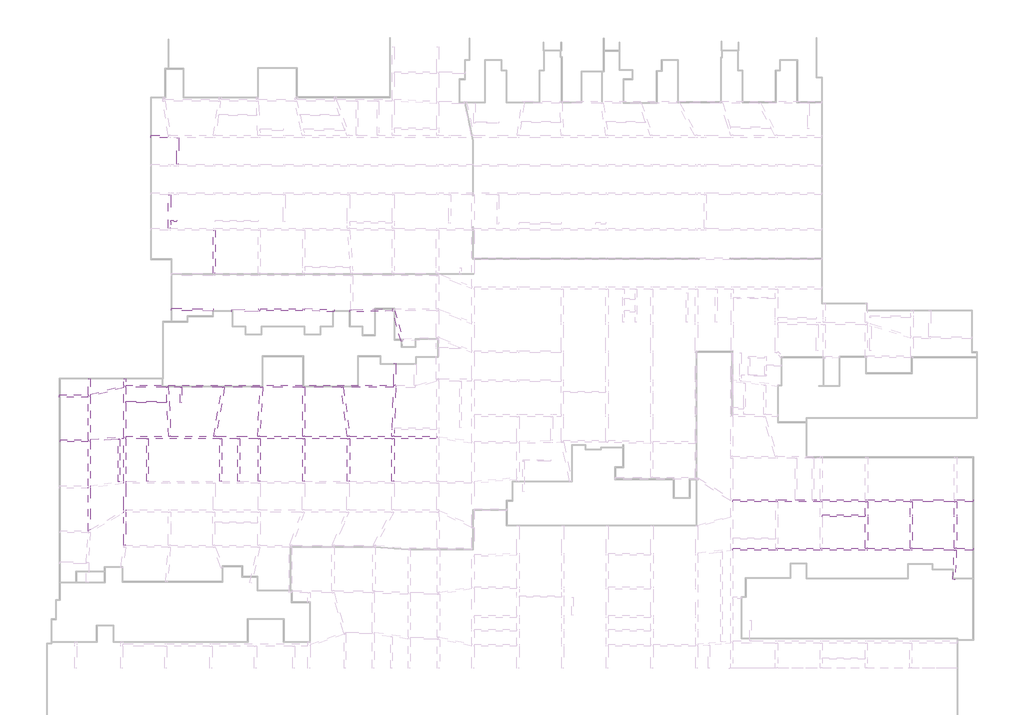
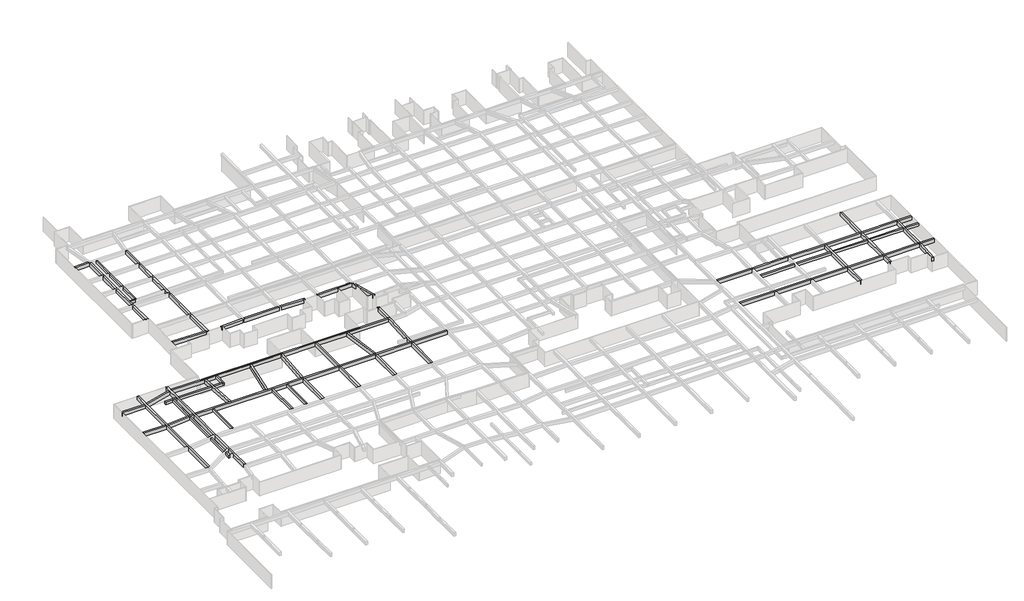
# One storey, part 11 of 16: 44 beams.
"""IFC4 building model written with IfcOpenShell, lengths in millimetres."""

from ifc_helpers import new_model, si_unit, frame, origin, place, context, project, spatial, polyline, outline, extrude, faceted_brep, element, save

model = new_model("IFC4")

# Units and contexts
model_context = context("Model", 3, world=origin())
ifc_project = project(units=[si_unit("LENGTHUNIT", "METRE", prefix="MILLI")], contexts=[model_context])

# Site, building, storey
site = spatial("IfcSite", under=ifc_project)
building = spatial("IfcBuilding", under=site)
storey = spatial("IfcBuildingStorey", under=building, Name="户型图", Elevation=0.0)

# Beams
placement = place(None, origin())
element("IfcBeam", 1, ObjectType="混凝土 - 矩形梁 : KL_beam", at=placement, inside=storey, context=model_context, shape_type="Brep", body=[
    faceted_brep([(83129.050114, 189895.7397162, 3300.0), (83129.050114, 190295.7397162, 3300.0), (83129.050114, 190295.7397162, 2500.0), (83129.050114, 189895.7397162, 2500.0), (86294.1615746, 189895.7397162, 3300.0), (86294.1615746, 190295.7397162, 3300.0), (86259.9916613, 190295.7397162, 3300.0), (86294.1615746, 190295.7397162, 2500.0), (86259.9916613, 190295.7397162, 2500.0), (86294.1615746, 189895.7397162, 2500.0)], [[[0, 1, 2, 3]], [[1, 0, 4, 5, 6]], [[2, 1, 6, 5, 7, 8]], [[3, 2, 8, 7, 9]], [[0, 3, 9, 4]], [[5, 4, 9, 7]]]),
])
element("IfcBeam", 2, ObjectType="混凝土 - 矩形梁 : KL_beam", at=placement, inside=storey, context=model_context, shape_type="Brep", body=[
    faceted_brep([(86694.1615746, 167850.6633594, 3300.0), (86294.1615746, 167850.6633594, 3300.0), (86294.1615746, 167850.6633594, 2500.0), (86694.1615746, 167850.6633594, 2500.0), (86694.1615746, 173112.5884701, 3300.0), (86294.1615746, 173112.5884701, 3300.0), (86294.1615746, 173112.5884701, 2500.0), (86694.1615746, 173112.5884701, 2500.0)], [[[0, 1, 2, 3]], [[1, 0, 4, 5]], [[2, 1, 5, 6]], [[3, 2, 6, 7]], [[0, 3, 7, 4]], [[5, 4, 7, 6]]]),
    faceted_brep([(86294.1615746, 189895.7397162, 3300.0), (86694.1615746, 189895.7397162, 3300.0), (86694.1615746, 189895.7397162, 2500.0), (86294.1615746, 189895.7397162, 2500.0), (86694.1615746, 185072.5884701, 3300.0), (86294.1615746, 185072.5884701, 3300.0), (86294.1615746, 185072.5884701, 2500.0), (86694.1615746, 185072.5884701, 2500.0)], [[[0, 1, 2, 3]], [[4, 5, 6, 7]], [[1, 0, 5, 4]], [[0, 3, 6, 5]], [[3, 2, 7, 6]], [[2, 1, 4, 7]]]),
    faceted_brep([(86294.1615746, 184672.5884701, 3300.0), (86694.1615746, 184672.5884701, 3300.0), (86694.1615746, 184672.5884701, 2500.0), (86294.1615746, 184672.5884701, 2500.0), (86694.1615746, 179912.5884701, 3300.0), (86294.1615746, 179912.5884701, 3300.0), (86294.1615746, 179912.5884701, 2500.0), (86694.1615746, 179912.5884701, 2500.0)], [[[0, 1, 2, 3]], [[4, 5, 6, 7]], [[1, 0, 5, 4]], [[0, 3, 6, 5]], [[3, 2, 7, 6]], [[2, 1, 4, 7]]]),
    faceted_brep([(86294.1615746, 179512.5884701, 3300.0), (86694.1615746, 179512.5884701, 3300.0), (86694.1615746, 179512.5884701, 2500.0), (86294.1615746, 179512.5884701, 2500.0), (86694.1615746, 173512.5884701, 3300.0), (86294.1615746, 173512.5884701, 3300.0), (86294.1615746, 173512.5884701, 2500.0), (86694.1615746, 173512.5884701, 2500.0), (86694.1615746, 174669.5403425, 3300.0), (86694.1615746, 174969.5403425, 3300.0)], [[[0, 1, 2, 3]], [[4, 5, 6, 7]], [[1, 0, 5, 4, 8, 9]], [[0, 3, 6, 5]], [[3, 2, 7, 6]], [[2, 1, 9, 8, 4, 7]]]),
])
element("IfcBeam", 3, ObjectType="混凝土 - 矩形梁 : KL_beam", at=placement, inside=storey, context=model_context, shape_type="Brep", body=[
    faceted_brep([(94416.2109037, 158476.0490175, 3300.0), (94816.2109037, 158476.0490175, 3300.0), (94816.2109037, 164912.5884701, 3300.0), (94416.2109037, 164912.5884701, 3300.0), (94416.2109037, 158876.1099487, 3300.0), (94416.2109037, 158476.0490175, 2500.0), (94416.2109037, 164912.5884701, 2500.0), (94416.2109037, 158876.1099487, 2500.0), (94816.2109037, 158476.0490175, 2500.0), (94816.2109037, 164912.5884701, 2500.0)], [[[0, 1, 2, 3, 4]], [[5, 0, 4, 3, 6, 7]], [[8, 5, 7, 6, 9]], [[1, 8, 9, 2]], [[3, 2, 9, 6]], [[1, 0, 5, 8]]]),
    faceted_brep([(94416.2109037, 189895.7397162, 3300.0), (94816.2109037, 189895.7397162, 3300.0), (94816.2109037, 189895.7397162, 2500.0), (94416.2109037, 189895.7397162, 2500.0), (94816.2109037, 185072.5884701, 3300.0), (94416.2109037, 185072.5884701, 3300.0), (94416.2109037, 185072.5884701, 2500.0), (94816.2109037, 185072.5884701, 2500.0)], [[[0, 1, 2, 3]], [[4, 5, 6, 7]], [[1, 0, 5, 4]], [[0, 3, 6, 5]], [[3, 2, 7, 6]], [[2, 1, 4, 7]]]),
    faceted_brep([(94416.2109037, 184672.5884701, 3300.0), (94816.2109037, 184672.5884701, 3300.0), (94816.2109037, 184672.5884701, 2500.0), (94416.2109037, 184672.5884701, 2500.0), (94816.2109037, 179912.5884701, 3300.0), (94416.2109037, 179912.5884701, 3300.0), (94416.2109037, 179912.5884701, 2500.0), (94816.2109037, 179912.5884701, 2500.0)], [[[0, 1, 2, 3]], [[4, 5, 6, 7]], [[1, 0, 5, 4]], [[0, 3, 6, 5]], [[3, 2, 7, 6]], [[2, 1, 4, 7]]]),
    faceted_brep([(94416.2109037, 179512.5884701, 3300.0), (94816.2109037, 179512.5884701, 3300.0), (94816.2109037, 179512.5884701, 2500.0), (94416.2109037, 179512.5884701, 2500.0), (94816.2109037, 173512.5884701, 3300.0), (94416.2109037, 173512.5884701, 3300.0), (94416.2109037, 173512.5884701, 2500.0), (94816.2109037, 173512.5884701, 2500.0), (94416.2109037, 174969.5403425, 3300.0), (94416.2109037, 174669.5403425, 3300.0), (94816.2109037, 174669.5403425, 3300.0), (94816.2109037, 174969.5403425, 3300.0)], [[[0, 1, 2, 3]], [[4, 5, 6, 7]], [[1, 0, 8, 9, 5, 4, 10, 11]], [[0, 3, 6, 5, 9, 8]], [[3, 2, 7, 6]], [[2, 1, 11, 10, 4, 7]]]),
    faceted_brep([(94416.2109037, 173112.5884701, 3300.0), (94816.2109037, 173112.5884701, 3300.0), (94816.2109037, 173112.5884701, 2500.0), (94416.2109037, 173112.5884701, 2500.0), (94816.2109037, 165312.5884701, 3300.0), (94416.2109037, 165312.5884701, 3300.0), (94416.2109037, 165312.5884701, 2500.0), (94816.2109037, 165312.5884701, 2500.0)], [[[0, 1, 2, 3]], [[4, 5, 6, 7]], [[1, 0, 5, 4]], [[0, 3, 6, 5]], [[3, 2, 7, 6]], [[2, 1, 4, 7]]]),
])
element("IfcBeam", 4, ObjectType="混凝土 - 矩形梁 : KL_beam", at=placement, inside=storey, context=model_context, shape_type="Brep", body=[
    faceted_brep([(86825.6773723, 158608.5422731, 3300.0), (86832.6583349, 159008.4813512, 3300.0), (86832.6583349, 159008.4813512, 2500.0), (86825.6773723, 158608.5422731, 2500.0), (94416.2109037, 158476.0490175, 3300.0), (94416.2109037, 158876.1099487, 3300.0), (94416.2109037, 158876.1099487, 2500.0), (94416.2109037, 158476.0490175, 2500.0), (94816.2109037, 158469.0669915, 2500.0), (94816.2109037, 158469.0669915, 3300.0), (94816.2109037, 158476.0490175, 2500.0), (94816.2109037, 158476.0490175, 3300.0)], [[[0, 1, 2, 3]], [[1, 0, 4, 5]], [[2, 1, 5, 6]], [[3, 2, 6, 7]], [[0, 3, 7, 8, 9, 4]], [[9, 8, 10, 11]], [[4, 7, 6, 5]], [[7, 4, 11, 10]], [[4, 9, 11]], [[10, 8, 7]]]),
])
element("IfcBeam", 5, ObjectType="混凝土 - 矩形梁 : KL_beam", at=placement, inside=storey, context=model_context, shape_type="SweptSolid", body=[
    extrude(outline(polyline([(97729.8525124, 158312.7245419), (97715.1918872, 158712.4557842), (102516.2109037, 158888.5389443), (102516.2109037, 158488.2700059), (97729.8525124, 158312.7245419)])), frame((0.0, 0.0, 2500.0), z_axis=(0.0, 0.0, 1.0), x_axis=(1.0, 0.0, 0.0)), (0.0, 0.0, 1.0), 800.0),
])
element("IfcBeam", 6, ObjectType="混凝土 - 矩形梁 : KL_beam", at=placement, inside=storey, context=model_context, shape_type="SweptSolid", body=[
    extrude(outline(polyline([(102916.2109037, 158502.9404881), (102916.2109037, 158895.7397162), (110616.2109037, 158895.7397162), (110616.2109037, 158495.7397162), (102719.8772917, 158495.7397162), (102916.2109037, 158502.9404881)])), frame((0.0, 0.0, 2500.0), z_axis=(0.0, 0.0, 1.0), x_axis=(1.0, 0.0, 0.0)), (0.0, 0.0, 1.0), 800.0),
])
element("IfcBeam", 7, ObjectType="混凝土 - 矩形梁 : KL_beam", at=placement, inside=storey, context=model_context, shape_type="SweptSolid", body=[
    extrude(outline(polyline([(116332.4791504, 158712.3385391), (116311.9369207, 158312.8663663), (111016.2109037, 158585.1907676), (111016.2109037, 158985.7192923), (116332.4791504, 158712.3385391)])), frame((0.0, 0.0, 2500.0), z_axis=(0.0, 0.0, 1.0), x_axis=(1.0, 0.0, 0.0)), (0.0, 0.0, 1.0), 800.0),
])
element("IfcBeam", 8, ObjectType="混凝土 - 矩形梁 : KL_beam", at=placement, inside=storey, context=model_context, shape_type="Brep", body=[
    faceted_brep([(119117.5153204, 158712.5269028, 3300.0), (119117.5153204, 158712.5269028, 2500.0), (119127.7719841, 158312.6584233, 2500.0), (119127.7719841, 158312.6584233, 3300.0), (126816.2109037, 158509.867597, 3300.0), (126816.2109037, 158909.9991608, 3300.0), (119689.6107616, 158727.2012041, 3300.0), (119289.6107616, 158716.9411668, 3300.0), (126816.2109037, 158509.867597, 2500.0), (119289.6107616, 158716.9411668, 2500.0), (119689.6107616, 158727.2012041, 2500.0), (126816.2109037, 158909.9991608, 2500.0)], [[[0, 1, 2, 3]], [[0, 3, 4, 5, 6, 7]], [[3, 2, 8, 4]], [[2, 1, 9, 10, 11, 8]], [[1, 0, 7, 6, 5, 11, 10, 9]], [[5, 4, 8, 11]]]),
])
element("IfcBeam", 9, ObjectType="混凝土 - 矩形梁 : KL_beam", at=placement, inside=storey, context=model_context, shape_type="Brep", body=[
    faceted_brep([(128438.9418632, 153027.8198438, 3300.0), (128848.9009007, 153049.3048866, 3300.0), (128735.7458004, 153443.9236175, 3300.0), (127281.619868, 158515.0633975, 3300.0), (127018.7754912, 158515.0633975, 3300.0), (126866.6192101, 158511.1605747, 3300.0), (126866.6192101, 158511.1605747, 2500.0), (128438.9418632, 153027.8198438, 2500.0), (128848.9009007, 153049.3048866, 2500.0), (127018.7754912, 158515.0633975, 2500.0), (127281.619868, 158515.0633975, 2500.0), (128735.7458004, 153443.9236175, 2500.0)], [[[0, 1, 2, 3, 4, 5]], [[5, 6, 7, 0]], [[8, 7, 6, 9, 10, 11]], [[1, 8, 11, 10, 3, 2]], [[6, 5, 4, 9]], [[4, 3, 10, 9]], [[1, 0, 7, 8]]]),
])
element("IfcBeam", 10, ObjectType="混凝土 - 矩形梁 : KL_beam", at=placement, inside=storey, context=model_context, shape_type="Brep", body=[
    faceted_brep([(232045.6960739, 124332.2101355, 3300.0), (232045.6960739, 123932.2101355, 3300.0), (232045.6960739, 123932.2101355, 2500.0), (232045.6960739, 124332.2101355, 2500.0), (229016.2421537, 124332.2101355, 3300.0), (228616.2421537, 124332.2101355, 3300.0), (221016.2265287, 124332.2101355, 3300.0), (220616.2265287, 124332.2101355, 3300.0), (212916.2109037, 124332.2101355, 3300.0), (212516.2109037, 124332.2101355, 3300.0), (204716.2109037, 124332.2101355, 3300.0), (204316.2109037, 124332.2101355, 3300.0), (203157.9308744, 124332.2101355, 3300.0), (202857.9308744, 124332.2101355, 3300.0), (200116.9298732, 124332.2101355, 3300.0), (199816.9298732, 124332.2101355, 3300.0), (196655.472134, 124332.2101355, 3300.0), (196255.472134, 124332.2101355, 3300.0), (188516.2109037, 124332.2101355, 3300.0), (188516.2109037, 123932.2101355, 3300.0), (196255.472134, 123932.2101355, 3300.0), (196655.472134, 123932.2101355, 3300.0), (204316.2109037, 123932.2101355, 3300.0), (204716.2109037, 123932.2101355, 3300.0), (212516.2109037, 123932.2101355, 3300.0), (212916.2109037, 123932.2101355, 3300.0), (220616.2265287, 123932.2101355, 3300.0), (221016.2265287, 123932.2101355, 3300.0), (228616.2421537, 123932.2101355, 3300.0), (229016.2421537, 123932.2101355, 3300.0), (188516.2109037, 123932.2101355, 2500.0), (196255.472134, 123932.2101355, 2500.0), (196655.472134, 123932.2101355, 2500.0), (204316.2109037, 123932.2101355, 2500.0), (204716.2109037, 123932.2101355, 2500.0), (212516.2109037, 123932.2101355, 2500.0), (212916.2109037, 123932.2101355, 2500.0), (220616.2265287, 123932.2101355, 2500.0), (221016.2265287, 123932.2101355, 2500.0), (228616.2421537, 123932.2101355, 2500.0), (229016.2421537, 123932.2101355, 2500.0), (188516.2109037, 124332.2101355, 2500.0), (196255.472134, 124332.2101355, 2500.0), (196655.472134, 124332.2101355, 2500.0), (204316.2109037, 124332.2101355, 2500.0), (204716.2109037, 124332.2101355, 2500.0), (212516.2109037, 124332.2101355, 2500.0), (212916.2109037, 124332.2101355, 2500.0), (220616.2265287, 124332.2101355, 2500.0), (221016.2265287, 124332.2101355, 2500.0), (228616.2421537, 124332.2101355, 2500.0), (229016.2421537, 124332.2101355, 2500.0)], [[[0, 1, 2, 3]], [[1, 0, 4, 5, 6, 7, 8, 9, 10, 11, 12, 13, 14, 15, 16, 17, 18, 19, 20, 21, 22, 23, 24, 25, 26, 27, 28, 29]], [[2, 1, 29, 28, 27, 26, 25, 24, 23, 22, 21, 20, 19, 30, 31, 32, 33, 34, 35, 36, 37, 38, 39, 40]], [[3, 2, 40, 39, 38, 37, 36, 35, 34, 33, 32, 31, 30, 41, 42, 43, 44, 45, 46, 47, 48, 49, 50, 51]], [[0, 3, 51, 50, 49, 48, 47, 46, 45, 44, 43, 42, 41, 18, 17, 16, 15, 14, 13, 12, 11, 10, 9, 8, 7, 6, 5, 4]], [[18, 41, 30, 19]]]),
])
element("IfcBeam", 11, ObjectType="混凝土 - 矩形梁 : KL_beam", at=placement, inside=storey, context=model_context, shape_type="Brep", body=[
    faceted_brep([(232047.570889, 115530.098028, 3300.0), (232047.570889, 115130.098028, 3300.0), (232047.570889, 115130.098028, 2500.0), (232047.570889, 115530.098028, 2500.0), (229016.2421537, 115530.098028, 3300.0), (228616.2421537, 115530.098028, 3300.0), (221016.2265287, 115530.098028, 3300.0), (220616.2265287, 115530.098028, 3300.0), (212916.2109037, 115530.098028, 3300.0), (212516.2109037, 115530.098028, 3300.0), (204716.2109037, 115530.098028, 3300.0), (204316.2109037, 115530.098028, 3300.0), (196655.472134, 115530.098028, 3300.0), (196255.472134, 115530.098028, 3300.0), (188516.2109037, 115530.098028, 3300.0), (188516.2109037, 115130.098028, 3300.0), (196255.472134, 115130.098028, 3300.0), (196655.472134, 115130.098028, 3300.0), (204316.2109037, 115130.098028, 3300.0), (204716.2109037, 115130.098028, 3300.0), (212516.2109037, 115130.098028, 3300.0), (212916.2109037, 115130.098028, 3300.0), (220616.2265287, 115130.098028, 3300.0), (221016.2265287, 115130.098028, 3300.0), (228606.1893059, 115130.098028, 3300.0), (229006.6704217, 115130.098028, 3300.0), (188516.2109037, 115130.098028, 2500.0), (196255.472134, 115130.098028, 2500.0), (196655.472134, 115130.098028, 2500.0), (204316.2109037, 115130.098028, 2500.0), (204716.2109037, 115130.098028, 2500.0), (212516.2109037, 115130.098028, 2500.0), (212916.2109037, 115130.098028, 2500.0), (220616.2265287, 115130.098028, 2500.0), (221016.2265287, 115130.098028, 2500.0), (228606.1893059, 115130.098028, 2500.0), (229006.6704217, 115130.098028, 2500.0), (188516.2109037, 115530.098028, 2500.0), (196255.472134, 115530.098028, 2500.0), (196655.472134, 115530.098028, 2500.0), (204316.2109037, 115530.098028, 2500.0), (204716.2109037, 115530.098028, 2500.0), (212516.2109037, 115530.098028, 2500.0), (212916.2109037, 115530.098028, 2500.0), (220616.2265287, 115530.098028, 2500.0), (221016.2265287, 115530.098028, 2500.0), (228616.2421537, 115530.098028, 2500.0), (229016.2421537, 115530.098028, 2500.0)], [[[0, 1, 2, 3]], [[1, 0, 4, 5, 6, 7, 8, 9, 10, 11, 12, 13, 14, 15, 16, 17, 18, 19, 20, 21, 22, 23, 24, 25]], [[2, 1, 25, 24, 23, 22, 21, 20, 19, 18, 17, 16, 15, 26, 27, 28, 29, 30, 31, 32, 33, 34, 35, 36]], [[3, 2, 36, 35, 34, 33, 32, 31, 30, 29, 28, 27, 26, 37, 38, 39, 40, 41, 42, 43, 44, 45, 46, 47]], [[0, 3, 47, 46, 45, 44, 43, 42, 41, 40, 39, 38, 37, 14, 13, 12, 11, 10, 9, 8, 7, 6, 5, 4]], [[15, 14, 37, 26]]]),
])
element("IfcBeam", 12, ObjectType="混凝土 - 矩形梁 : KL_beam", at=placement, inside=storey, context=model_context, shape_type="Brep", body=[
    faceted_brep([(212916.2109037, 110061.7118028, 3300.0), (212516.2109037, 110061.7118028, 3300.0), (212516.2109037, 110061.7118028, 2500.0), (212916.2109037, 110061.7118028, 2500.0), (212916.2109037, 115130.098028, 3300.0), (212516.2109037, 115130.098028, 3300.0), (212516.2109037, 115130.098028, 2500.0), (212916.2109037, 115130.098028, 2500.0)], [[[0, 1, 2, 3]], [[1, 0, 4, 5]], [[2, 1, 5, 6]], [[3, 2, 6, 7]], [[0, 3, 7, 4]], [[5, 4, 7, 6]]]),
    faceted_brep([(212516.2109037, 123932.2101355, 3300.0), (212916.2109037, 123932.2101355, 3300.0), (212916.2109037, 123932.2101355, 2500.0), (212516.2109037, 123932.2101355, 2500.0), (212916.2109037, 115530.098028, 3300.0), (212516.2109037, 115530.098028, 3300.0), (212516.2109037, 115530.098028, 2500.0), (212916.2109037, 115530.098028, 2500.0), (212516.2109037, 121562.5884701, 3300.0), (212516.2109037, 121262.5884701, 3300.0), (212916.2109037, 121262.5884701, 3300.0), (212916.2109037, 121562.5884701, 3300.0)], [[[0, 1, 2, 3]], [[4, 5, 6, 7]], [[1, 0, 8, 9, 5, 4, 10, 11]], [[0, 3, 6, 5, 9, 8]], [[3, 2, 7, 6]], [[2, 1, 11, 10, 4, 7]]]),
])
element("IfcBeam", 13, ObjectType="混凝土 - 矩形梁 : KL_beam", at=placement, inside=storey, context=model_context, shape_type="Brep", body=[
    faceted_brep([(221016.2265287, 112661.2598568, 3300.0), (220616.2265287, 112661.2598568, 3300.0), (220616.2265287, 112661.2598568, 2500.0), (221016.2265287, 112661.2598568, 2500.0), (221016.2265287, 115130.098028, 3300.0), (220616.2265287, 115130.098028, 3300.0), (220616.2265287, 115130.098028, 2500.0), (221016.2265287, 115130.098028, 2500.0)], [[[0, 1, 2, 3]], [[1, 0, 4, 5]], [[2, 1, 5, 6]], [[3, 2, 6, 7]], [[0, 3, 7, 4]], [[5, 4, 7, 6]]]),
    faceted_brep([(221016.2265287, 132011.2598568, 3300.0), (221016.2265287, 132011.2598568, 2500.0), (220616.2265287, 132011.2598568, 2500.0), (220616.2265287, 132011.2598568, 3300.0), (221016.2265287, 124332.2101355, 3300.0), (220616.2265287, 124332.2101355, 3300.0), (220616.2265287, 124332.2101355, 2500.0), (221016.2265287, 124332.2101355, 2500.0)], [[[0, 1, 2, 3]], [[4, 5, 6, 7]], [[0, 3, 5, 4]], [[3, 2, 6, 5]], [[2, 1, 7, 6]], [[1, 0, 4, 7]]]),
    faceted_brep([(220616.2265287, 123932.2101355, 3300.0), (221016.2265287, 123932.2101355, 3300.0), (221016.2265287, 123932.2101355, 2500.0), (220616.2265287, 123932.2101355, 2500.0), (221016.2265287, 115530.098028, 3300.0), (220616.2265287, 115530.098028, 3300.0), (220616.2265287, 115530.098028, 2500.0), (221016.2265287, 115530.098028, 2500.0), (220616.2265287, 121562.5884701, 3300.0), (220616.2265287, 121262.5884701, 3300.0), (221016.2265287, 121262.5884701, 3300.0), (221016.2265287, 121562.5884701, 3300.0)], [[[0, 1, 2, 3]], [[4, 5, 6, 7]], [[1, 0, 8, 9, 5, 4, 10, 11]], [[0, 3, 6, 5, 9, 8]], [[3, 2, 7, 6]], [[2, 1, 11, 10, 4, 7]]]),
])
element("IfcBeam", 14, ObjectType="混凝土 - 矩形梁 : KL_beam", at=placement, inside=storey, context=model_context, shape_type="Brep", body=[
    faceted_brep([(229016.2421537, 123932.2101355, 3300.0), (228616.2421537, 123932.2101355, 3300.0), (228616.2421537, 121562.5884701, 3300.0), (228616.2421537, 121262.5884701, 3300.0), (228616.2421537, 115530.098028, 3300.0), (229016.2421537, 115530.098028, 3300.0), (229016.2421537, 121262.5884701, 3300.0), (229016.2421537, 121562.5884701, 3300.0), (228616.2421537, 123932.2101355, 2500.0), (228616.2421537, 115530.098028, 2500.0), (229016.2421537, 123932.2101355, 2500.0), (229016.2421537, 115530.098028, 2500.0)], [[[0, 1, 2, 3, 4, 5, 6, 7]], [[1, 8, 9, 4, 3, 2]], [[8, 10, 11, 9]], [[10, 0, 7, 6, 5, 11]], [[1, 0, 10, 8]], [[5, 4, 9, 11]]]),
])
element("IfcBeam", 15, ObjectType="混凝土 - 矩形梁 : KL_beam", at=placement, inside=storey, context=model_context, shape_type="SweptSolid", body=[
    extrude(outline(polyline([(228747.7018146, 109851.643928), (228348.1823524, 109871.2449317), (228606.1893059, 115130.098028), (229006.6704217, 115130.098028), (228747.7018146, 109851.643928)])), frame((0.0, 0.0, 2500.0), z_axis=(0.0, 0.0, 1.0), x_axis=(1.0, 0.0, 0.0)), (0.0, 0.0, 1.0), 800.0),
])
element("IfcBeam", 16, ObjectType="混凝土 - 矩形梁 : KL_beam", at=placement, inside=storey, context=model_context, shape_type="Brep", body=[
    faceted_brep([(78576.3134091, 135771.3777961, 3300.0), (78576.3134091, 135371.3777961, 3300.0), (82366.2109037, 135371.3777961, 3300.0), (82666.2109037, 135371.3777961, 3300.0), (95616.2109037, 135371.3777961, 3300.0), (95916.2109037, 135371.3777961, 3300.0), (98891.2109037, 135371.3777961, 3300.0), (99191.2109037, 135371.3777961, 3300.0), (102516.2109037, 135371.3777961, 3300.0), (102916.2109037, 135371.3777961, 3300.0), (110616.2109037, 135371.3777961, 3300.0), (111016.2109037, 135371.3777961, 3300.0), (118712.9467119, 135371.3777961, 3300.0), (119112.9467119, 135371.3777961, 3300.0), (126752.364693, 135371.3777961, 3300.0), (127152.364693, 135371.3777961, 3300.0), (134872.1367776, 135371.3777961, 3300.0), (134872.1367776, 135771.3777961, 3300.0), (127159.4707558, 135771.3777961, 3300.0), (126759.2269381, 135771.3777961, 3300.0), (119089.8917648, 135771.3777961, 3300.0), (118686.8878346, 135771.3777961, 3300.0), (111016.2109037, 135771.3777961, 3300.0), (110616.2109037, 135771.3777961, 3300.0), (102828.5469768, 135771.3777961, 3300.0), (102427.8302889, 135771.3777961, 3300.0), (94873.0389146, 135771.3777961, 3300.0), (94466.8682698, 135771.3777961, 3300.0), (86749.5721447, 135771.3777961, 3300.0), (86349.0232063, 135771.3777961, 3300.0), (78576.3134091, 135371.3777961, 2500.0), (102516.2109037, 135371.3777961, 2500.0), (102916.2109037, 135371.3777961, 2500.0), (110616.2109037, 135371.3777961, 2500.0), (111016.2109037, 135371.3777961, 2500.0), (118712.9467119, 135371.3777961, 2500.0), (119112.9467119, 135371.3777961, 2500.0), (126752.364693, 135371.3777961, 2500.0), (127152.364693, 135371.3777961, 2500.0), (134872.1367776, 135371.3777961, 2500.0), (78576.3134091, 135771.3777961, 2500.0), (86349.0232063, 135771.3777961, 2500.0), (86749.5721447, 135771.3777961, 2500.0), (94466.8682698, 135771.3777961, 2500.0), (94873.0389146, 135771.3777961, 2500.0), (102427.8302889, 135771.3777961, 2500.0), (102828.5469768, 135771.3777961, 2500.0), (110616.2109037, 135771.3777961, 2500.0), (111016.2109037, 135771.3777961, 2500.0), (118686.8878346, 135771.3777961, 2500.0), (119089.8917648, 135771.3777961, 2500.0), (126759.2269381, 135771.3777961, 2500.0), (127159.4707558, 135771.3777961, 2500.0), (134872.1367776, 135771.3777961, 2500.0)], [[[0, 1, 2, 3, 4, 5, 6, 7, 8, 9, 10, 11, 12, 13, 14, 15, 16, 17, 18, 19, 20, 21, 22, 23, 24, 25, 26, 27, 28, 29]], [[1, 30, 31, 32, 33, 34, 35, 36, 37, 38, 39, 16, 15, 14, 13, 12, 11, 10, 9, 8, 7, 6, 5, 4, 3, 2]], [[30, 40, 41, 42, 43, 44, 45, 46, 47, 48, 49, 50, 51, 52, 53, 39, 38, 37, 36, 35, 34, 33, 32, 31]], [[40, 0, 29, 28, 27, 26, 25, 24, 23, 22, 21, 20, 19, 18, 17, 53, 52, 51, 50, 49, 48, 47, 46, 45, 44, 43, 42, 41]], [[1, 0, 40, 30]], [[17, 16, 39, 53]]]),
])
element("IfcBeam", 17, ObjectType="混凝土 - 矩形梁 : KL_beam", at=placement, inside=storey, context=model_context, shape_type="Brep", body=[
    faceted_brep([(78576.3134091, 146262.0423748, 3300.0), (78576.3134091, 146262.0423748, 2500.0), (78176.3134091, 146262.0423748, 2500.0), (78176.3134091, 146262.0423748, 3300.0), (78176.3134091, 145022.2074733, 3300.0), (78176.3134091, 144607.4530358, 3300.0), (78176.3134091, 142166.4564837, 3300.0), (78176.3134091, 141866.4564837, 3300.0), (78176.3134091, 135754.7019056, 3300.0), (78176.3134091, 135353.1850002, 3300.0), (78176.3134091, 127667.9134655, 3300.0), (78176.3134091, 127264.1539482, 3300.0), (78176.3134091, 122400.1381649, 3300.0), (78176.3134091, 121936.5309598, 3300.0), (78176.3134091, 120366.4564837, 3300.0), (78176.3134091, 120066.4564837, 3300.0), (78176.3134091, 116076.7662248, 3300.0), (78576.3134091, 116076.7662248, 3300.0), (78576.3134091, 120066.4564837, 3300.0), (78576.3134091, 120366.4564837, 3300.0), (78576.3134091, 122085.5220623, 3300.0), (78576.3134091, 122485.5220623, 3300.0), (78576.3134091, 127293.5189202, 3300.0), (78576.3134091, 127693.5189202, 3300.0), (78576.3134091, 135371.3777961, 3300.0), (78576.3134091, 135771.3777961, 3300.0), (78576.3134091, 141866.4564837, 3300.0), (78576.3134091, 142166.4564837, 3300.0), (78576.3134091, 144669.6509701, 3300.0), (78576.3134091, 145069.6509701, 3300.0), (78176.3134091, 145022.2074733, 2500.0), (78176.3134091, 144607.4530358, 2500.0), (78176.3134091, 135754.7019056, 2500.0), (78176.3134091, 135353.1850002, 2500.0), (78176.3134091, 127667.9134655, 2500.0), (78176.3134091, 127264.1539482, 2500.0), (78176.3134091, 122400.1381649, 2500.0), (78176.3134091, 121936.5309598, 2500.0), (78176.3134091, 116076.7662248, 2500.0), (78576.3134091, 145069.6509701, 2500.0), (78576.3134091, 144669.6509701, 2500.0), (78576.3134091, 135771.3777961, 2500.0), (78576.3134091, 135371.3777961, 2500.0), (78576.3134091, 127693.5189202, 2500.0), (78576.3134091, 127293.5189202, 2500.0), (78576.3134091, 122485.5220623, 2500.0), (78576.3134091, 122085.5220623, 2500.0), (78576.3134091, 116076.7662248, 2500.0)], [[[0, 1, 2, 3]], [[0, 3, 4, 5, 6, 7, 8, 9, 10, 11, 12, 13, 14, 15, 16, 17, 18, 19, 20, 21, 22, 23, 24, 25, 26, 27, 28, 29]], [[3, 2, 30, 31, 32, 33, 34, 35, 36, 37, 38, 16, 15, 14, 13, 12, 11, 10, 9, 8, 7, 6, 5, 4]], [[2, 1, 39, 40, 41, 42, 43, 44, 45, 46, 47, 38, 37, 36, 35, 34, 33, 32, 31, 30]], [[1, 0, 29, 28, 27, 26, 25, 24, 23, 22, 21, 20, 19, 18, 17, 47, 46, 45, 44, 43, 42, 41, 40, 39]], [[17, 16, 38, 47]]]),
])
element("IfcBeam", 18, ObjectType="混凝土 - 矩形梁 : KL_beam", at=placement, inside=storey, context=model_context, shape_type="Brep", body=[
    faceted_brep([(86283.2334082, 144669.6509701, 3300.0), (86262.2702965, 145069.6509701, 3300.0), (78576.3134091, 145069.6509701, 3300.0), (78576.3134091, 144669.6509701, 3300.0), (85882.6844698, 144669.6509701, 3300.0), (86283.2334082, 144669.6509701, 2500.0), (78576.3134091, 144669.6509701, 2500.0), (85882.6844698, 144669.6509701, 2500.0), (86262.2702965, 145069.6509701, 2500.0), (78576.3134091, 145069.6509701, 2500.0)], [[[0, 1, 2, 3, 4]], [[5, 0, 4, 3, 6, 7]], [[8, 5, 7, 6, 9]], [[1, 8, 9, 2]], [[3, 2, 9, 6]], [[1, 0, 5, 8]]]),
])
element("IfcBeam", 19, ObjectType="混凝土 - 矩形梁 : KL_beam", at=placement, inside=storey, context=model_context, shape_type="Brep", body=[
    faceted_brep([(86283.2334082, 144669.6509701, 3300.0), (85882.6844698, 144669.6509701, 3300.0), (86013.871334, 142166.4564837, 3300.0), (86029.5936677, 141866.4564837, 3300.0), (86349.0232063, 135771.3777961, 3300.0), (86749.5721447, 135771.3777961, 3300.0), (86430.1426061, 141866.4564837, 3300.0), (86414.4202724, 142166.4564837, 3300.0), (85882.6844698, 144669.6509701, 2500.0), (86349.0232063, 135771.3777961, 2500.0), (86283.2334082, 144669.6509701, 2500.0), (86749.5721447, 135771.3777961, 2500.0)], [[[0, 1, 2, 3, 4, 5, 6, 7]], [[1, 8, 9, 4, 3, 2]], [[8, 10, 11, 9]], [[10, 0, 7, 6, 5, 11]], [[1, 0, 10, 8]], [[5, 4, 9, 11]]]),
])
element("IfcBeam", 20, ObjectType="混凝土 - 矩形梁 : KL_beam", at=placement, inside=storey, context=model_context, shape_type="SweptSolid", body=[
    extrude(outline(polyline([(94873.0389146, 135771.3777961), (94466.8682698, 135771.3777961), (96035.8739121, 144669.6509701), (96442.0445569, 144669.6509701), (94873.0389146, 135771.3777961)])), frame((0.0, 0.0, 2500.0), z_axis=(0.0, 0.0, 1.0), x_axis=(1.0, 0.0, 0.0)), (0.0, 0.0, 1.0), 800.0),
])
element("IfcBeam", 21, ObjectType="混凝土 - 矩形梁 : KL_beam", at=placement, inside=storey, context=model_context, shape_type="SweptSolid", body=[
    extrude(outline(polyline([(102828.5469768, 135771.3777961), (102427.8302889, 135771.3777961), (102960.735821, 144669.6509701), (103361.4525089, 144669.6509701), (102828.5469768, 135771.3777961)])), frame((0.0, 0.0, 2500.0), z_axis=(0.0, 0.0, 1.0), x_axis=(1.0, 0.0, 0.0)), (0.0, 0.0, 1.0), 800.0),
])
element("IfcBeam", 22, ObjectType="混凝土 - 矩形梁 : KL_beam", at=placement, inside=storey, context=model_context, shape_type="SweptSolid", body=[
    extrude(outline(polyline([(111016.2109037, 135771.3777961), (110616.2109037, 135771.3777961), (110616.2109037, 144669.6509701), (111016.2109037, 144669.6509701), (111016.2109037, 135771.3777961)])), frame((0.0, 0.0, 2500.0), z_axis=(0.0, 0.0, 1.0), x_axis=(1.0, 0.0, 0.0)), (0.0, 0.0, 1.0), 800.0),
])
element("IfcBeam", 23, ObjectType="混凝土 - 矩形梁 : KL_beam", at=placement, inside=storey, context=model_context, shape_type="SweptSolid", body=[
    extrude(outline(polyline([(102516.2109037, 135371.3777961), (102916.2109037, 135371.3777961), (102916.2109037, 127693.5189202), (102516.2109037, 127693.5189202), (102516.2109037, 135371.3777961)])), frame((0.0, 0.0, 2500.0), z_axis=(0.0, 0.0, 1.0), x_axis=(1.0, 0.0, 0.0)), (0.0, 0.0, 1.0), 800.0),
])
element("IfcBeam", 24, ObjectType="混凝土 - 矩形梁 : KL_beam", at=placement, inside=storey, context=model_context, shape_type="SweptSolid", body=[
    extrude(outline(polyline([(110616.2109037, 135371.3777961), (111016.2109037, 135371.3777961), (111016.2109037, 127693.5189202), (110616.2109037, 127693.5189202), (110616.2109037, 135371.3777961)])), frame((0.0, 0.0, 2500.0), z_axis=(0.0, 0.0, 1.0), x_axis=(1.0, 0.0, 0.0)), (0.0, 0.0, 1.0), 800.0),
])
element("IfcBeam", 25, ObjectType="混凝土 - 矩形梁 : KL_beam", at=placement, inside=storey, context=model_context, shape_type="SweptSolid", body=[
    extrude(outline(polyline([(119089.8917648, 135771.3777961), (118686.8878346, 135771.3777961), (117594.3172702, 144669.6509701), (117997.3212003, 144669.6509701), (119089.8917648, 135771.3777961)])), frame((0.0, 0.0, 2500.0), z_axis=(0.0, 0.0, 1.0), x_axis=(1.0, 0.0, 0.0)), (0.0, 0.0, 1.0), 800.0),
])
element("IfcBeam", 26, ObjectType="混凝土 - 矩形梁 : KL_beam", at=placement, inside=storey, context=model_context, shape_type="Brep", body=[
    faceted_brep([(127482.2091287, 145013.3955863, 3300.0), (127475.1030659, 145013.3955863, 3300.0), (127081.965311, 145013.3955863, 3300.0), (127075.1030659, 144816.8865993, 3300.0), (127069.9614845, 144669.6509701, 3300.0), (126813.4099874, 137322.9773199, 3300.0), (126802.9337565, 137022.9773199, 3300.0), (126759.2269381, 135771.3777961, 3300.0), (127159.4707558, 135771.3777961, 3300.0), (127203.1775743, 137022.9773199, 3300.0), (127213.6538051, 137322.9773199, 3300.0), (127468.2408209, 144613.3955863, 3300.0), (127081.965311, 145013.3955863, 2500.0), (127075.1030659, 144816.8865993, 2500.0), (127069.9614845, 144669.6509701, 2500.0), (126759.2269381, 135771.3777961, 2500.0), (127475.1030659, 145013.3955863, 2500.0), (127482.2091287, 145013.3955863, 2500.0), (127468.2408209, 144613.3955863, 2500.0), (127159.4707558, 135771.3777961, 2500.0)], [[[0, 1, 2, 3, 4, 5, 6, 7, 8, 9, 10, 11]], [[2, 12, 13, 14, 15, 7, 6, 5, 4, 3]], [[12, 16, 17, 18, 19, 15, 14, 13]], [[17, 0, 11, 10, 9, 8, 19, 18]], [[8, 7, 15, 19]], [[2, 1, 0, 17, 16, 12]]]),
])
element("IfcBeam", 27, ObjectType="混凝土 - 矩形梁 : KL_beam", at=placement, inside=storey, context=model_context, shape_type="SweptSolid", body=[
    extrude(outline(polyline([(118712.9467119, 135371.3777961), (119112.9467119, 135371.3777961), (119112.9467119, 127693.5189202), (118712.9467119, 127693.5189202), (118712.9467119, 135371.3777961)])), frame((0.0, 0.0, 2500.0), z_axis=(0.0, 0.0, 1.0), x_axis=(1.0, 0.0, 0.0)), (0.0, 0.0, 1.0), 800.0),
])
element("IfcBeam", 28, ObjectType="混凝土 - 矩形梁 : KL_beam", at=placement, inside=storey, context=model_context, shape_type="SweptSolid", body=[
    extrude(outline(polyline([(126752.364693, 135371.3777961), (127152.364693, 135371.3777961), (127152.364693, 127693.5189202), (126752.364693, 127693.5189202), (126752.364693, 135371.3777961)])), frame((0.0, 0.0, 2500.0), z_axis=(0.0, 0.0, 1.0), x_axis=(1.0, 0.0, 0.0)), (0.0, 0.0, 1.0), 800.0),
])
element("IfcBeam", 29, ObjectType="混凝土 - 矩形梁 : KL_beam", at=placement, inside=storey, context=model_context, shape_type="Brep", body=[
    faceted_brep([(127075.1030659, 149009.5233306, 3300.0), (127475.1030659, 149009.5233306, 3300.0), (127475.1030659, 149009.5233306, 2500.0), (127075.1030659, 149009.5233306, 2500.0), (127075.1030659, 145069.6509701, 3300.0), (127075.1030659, 144816.8865993, 3300.0), (127081.965311, 145013.3955863, 3300.0), (127475.1030659, 145013.3955863, 3300.0), (127475.1030659, 145013.3955863, 2500.0), (127081.965311, 145013.3955863, 2500.0), (127075.1030659, 144816.8865993, 2500.0), (127075.1030659, 145069.6509701, 2500.0)], [[[0, 1, 2, 3]], [[1, 0, 4, 5, 6, 7]], [[2, 1, 7, 8]], [[3, 2, 8, 9, 10, 11]], [[0, 3, 11, 10, 5, 4]], [[9, 6, 5, 10]], [[6, 9, 8, 7]]]),
])
element("IfcBeam", 30, ObjectType="混凝土 - 矩形梁 : KL_beam", at=placement, inside=storey, context=model_context, shape_type="Brep", body=[
    faceted_brep([(86262.2702965, 145069.6509701, 3300.0), (86283.2334082, 144669.6509701, 3300.0), (88422.554673, 144669.6509701, 3300.0), (88722.554673, 144669.6509701, 3300.0), (96035.8739121, 144669.6509701, 3300.0), (96442.0445569, 144669.6509701, 3300.0), (102960.735821, 144669.6509701, 3300.0), (103361.4525089, 144669.6509701, 3300.0), (110616.2109037, 144669.6509701, 3300.0), (111016.2109037, 144669.6509701, 3300.0), (117594.3172702, 144669.6509701, 3300.0), (117997.3212003, 144669.6509701, 3300.0), (127069.9614845, 144669.6509701, 3300.0), (127075.1030659, 144816.8865993, 3300.0), (127075.1030659, 145069.6509701, 3300.0), (86283.2334082, 144669.6509701, 2500.0), (96035.8739121, 144669.6509701, 2500.0), (96442.0445569, 144669.6509701, 2500.0), (102960.735821, 144669.6509701, 2500.0), (103361.4525089, 144669.6509701, 2500.0), (110616.2109037, 144669.6509701, 2500.0), (111016.2109037, 144669.6509701, 2500.0), (117594.3172702, 144669.6509701, 2500.0), (117997.3212003, 144669.6509701, 2500.0), (127069.9614845, 144669.6509701, 2500.0), (86262.2702965, 145069.6509701, 2500.0), (127075.1030659, 145069.6509701, 2500.0), (127075.1030659, 144816.8865993, 2500.0)], [[[0, 1, 2, 3, 4, 5, 6, 7, 8, 9, 10, 11, 12, 13, 14]], [[1, 15, 16, 17, 18, 19, 20, 21, 22, 23, 24, 12, 11, 10, 9, 8, 7, 6, 5, 4, 3, 2]], [[15, 25, 26, 27, 24, 23, 22, 21, 20, 19, 18, 17, 16]], [[25, 0, 14, 26]], [[1, 0, 25, 15]], [[12, 24, 27, 13]], [[14, 13, 27, 26]]]),
])
element("IfcBeam", 31, ObjectType="混凝土 - 矩形梁 : KL_beam", at=placement, inside=storey, context=model_context, shape_type="SweptSolid", body=[
    extrude(outline(polyline([(78176.3134091, 145022.2074733), (78176.3134091, 144607.4530358), (72166.4204182, 142960.1198643), (72166.4204182, 143374.8743018), (78176.3134091, 145022.2074733)])), frame((0.0, 0.0, 2500.0), z_axis=(0.0, 0.0, 1.0), x_axis=(1.0, 0.0, 0.0)), (0.0, 0.0, 1.0), 800.0),
])
element("IfcBeam", 32, ObjectType="混凝土 - 矩形梁 : KL_beam", at=placement, inside=storey, context=model_context, shape_type="Brep", body=[
    faceted_brep([(78176.3134091, 135353.1850002, 3300.0), (78176.3134091, 135754.7019056, 3300.0), (77490.6700269, 135694.9331952, 3300.0), (77190.6700269, 135668.7816804, 3300.0), (72166.4204182, 135230.8092196, 3300.0), (72166.4204182, 134829.2923142, 3300.0), (77190.6700269, 135267.264775, 3300.0), (77490.6700269, 135293.4162899, 3300.0), (78176.3134091, 135754.7019056, 2500.0), (72166.4204182, 135230.8092196, 2500.0), (78176.3134091, 135353.1850002, 2500.0), (72166.4204182, 134829.2923142, 2500.0)], [[[0, 1, 2, 3, 4, 5, 6, 7]], [[1, 8, 9, 4, 3, 2]], [[8, 10, 11, 9]], [[10, 0, 7, 6, 5, 11]], [[1, 0, 10, 8]], [[5, 4, 9, 11]]]),
])
element("IfcBeam", 33, ObjectType="混凝土 - 矩形梁 : KL_beam", at=placement, inside=storey, context=model_context, shape_type="Brep", body=[
    faceted_brep([(72166.4204182, 146262.0219564, 3300.0), (72166.4204182, 146262.0219564, 2500.0), (71766.4204182, 146262.0219564, 2500.0), (71766.4204182, 146262.0219564, 3300.0), (71766.4204182, 143312.6763675, 3300.0), (71766.4204182, 142912.6763675, 3300.0), (71766.4204182, 135212.6164237, 3300.0), (71766.4204182, 134812.6164237, 3300.0), (71766.4204182, 126812.6325388, 3300.0), (71766.4204182, 126412.6325388, 3300.0), (71766.4204182, 118729.7253879, 3300.0), (71766.4204182, 118644.3414905, 3300.0), (72166.4204182, 118878.7164905, 3300.0), (72166.4204182, 126438.2379935, 3300.0), (72166.4204182, 126841.9975108, 3300.0), (72166.4204182, 134829.2923142, 3300.0), (72166.4204182, 135230.8092196, 3300.0), (72166.4204182, 142960.1198643, 3300.0), (72166.4204182, 143374.8743018, 3300.0), (71766.4204182, 143312.6763675, 2500.0), (71766.4204182, 142912.6763675, 2500.0), (71766.4204182, 135212.6164237, 2500.0), (71766.4204182, 134812.6164237, 2500.0), (71766.4204182, 126812.6325388, 2500.0), (71766.4204182, 126412.6325388, 2500.0), (71766.4204182, 118729.7253879, 2500.0), (71766.4204182, 118644.3414905, 2500.0), (72166.4204182, 143374.8743018, 2500.0), (72166.4204182, 142960.1198643, 2500.0), (72166.4204182, 135230.8092196, 2500.0), (72166.4204182, 134829.2923142, 2500.0), (72166.4204182, 126841.9975108, 2500.0), (72166.4204182, 126438.2379935, 2500.0), (72166.4204182, 118878.7164905, 2500.0)], [[[0, 1, 2, 3]], [[0, 3, 4, 5, 6, 7, 8, 9, 10, 11, 12, 13, 14, 15, 16, 17, 18]], [[3, 2, 19, 20, 21, 22, 23, 24, 25, 26, 11, 10, 9, 8, 7, 6, 5, 4]], [[2, 1, 27, 28, 29, 30, 31, 32, 33, 26, 25, 24, 23, 22, 21, 20, 19]], [[1, 0, 18, 17, 16, 15, 14, 13, 12, 33, 32, 31, 30, 29, 28, 27]], [[12, 11, 26, 33]]]),
])
element("IfcBeam", 34, ObjectType="混凝土 - 矩形梁 : KL_beam", at=placement, inside=storey, context=model_context, shape_type="SweptSolid", body=[
    extrude(outline(polyline([(66666.4204182, 134812.6164237), (66666.4204182, 135212.6164237), (71766.4204182, 135212.6164237), (71766.4204182, 134812.6164237), (66666.4204182, 134812.6164237)])), frame((0.0, 0.0, 2500.0), z_axis=(0.0, 0.0, 1.0), x_axis=(1.0, 0.0, 0.0)), (0.0, 0.0, 1.0), 800.0),
])
element("IfcBeam", 35, ObjectType="混凝土 - 矩形梁 : KL_beam", at=placement, inside=storey, context=model_context, shape_type="SweptSolid", body=[
    extrude(outline(polyline([(66566.4204182, 142912.6763675), (66566.4204182, 143312.6763675), (71766.4204182, 143312.6763675), (71766.4204182, 142912.6763675), (66566.4204182, 142912.6763675)])), frame((0.0, 0.0, 2500.0), z_axis=(0.0, 0.0, 1.0), x_axis=(1.0, 0.0, 0.0)), (0.0, 0.0, 1.0), 800.0),
])
element("IfcBeam", 36, ObjectType="混凝土 - 矩形梁 : L_beam", at=placement, inside=storey, context=model_context, shape_type="SweptSolid", body=[
    extrude(outline(polyline([(88120.783903, 174969.5403425), (87820.783903, 174969.5403425), (87820.783903, 179512.5884701), (88120.783903, 179512.5884701), (88120.783903, 174969.5403425)])), frame((0.0, 0.0, 2700.0), z_axis=(0.0, 0.0, 1.0), x_axis=(1.0, 0.0, 0.0)), (0.0, 0.0, 1.0), 600.0),
    extrude(outline(polyline([(87820.783903, 189895.7397162), (88120.783903, 189895.7397162), (88120.783903, 185072.5884701), (87820.783903, 185072.5884701), (87820.783903, 189895.7397162)])), frame((0.0, 0.0, 2700.0), z_axis=(0.0, 0.0, 1.0), x_axis=(1.0, 0.0, 0.0)), (0.0, 0.0, 1.0), 600.0),
    extrude(outline(polyline([(87820.783903, 184672.5884701), (88120.783903, 184672.5884701), (88120.783903, 179912.5884701), (87820.783903, 179912.5884701), (87820.783903, 184672.5884701)])), frame((0.0, 0.0, 2700.0), z_axis=(0.0, 0.0, 1.0), x_axis=(1.0, 0.0, 0.0)), (0.0, 0.0, 1.0), 600.0),
])
element("IfcBeam", 37, ObjectType="混凝土 - 矩形梁 : L_beam", at=placement, inside=storey, context=model_context, shape_type="SweptSolid", body=[
    extrude(outline(polyline([(87820.783903, 174969.5403425), (87820.783903, 174669.5403425), (86694.1615746, 174669.5403425), (86694.1615746, 174969.5403425), (87820.783903, 174969.5403425)])), frame((0.0, 0.0, 2700.0), z_axis=(0.0, 0.0, 1.0), x_axis=(1.0, 0.0, 0.0)), (0.0, 0.0, 1.0), 600.0),
])
element("IfcBeam", 38, ObjectType="混凝土 - 矩形梁 : L_beam", at=placement, inside=storey, context=model_context, shape_type="Brep", body=[
    faceted_brep([(88422.554673, 141866.4564837, 3300.0), (88722.554673, 141866.4564837, 3300.0), (88722.554673, 144669.6509701, 3300.0), (88422.554673, 144669.6509701, 3300.0), (88422.554673, 142166.4564837, 3300.0), (88422.554673, 141866.4564837, 2700.0), (88422.554673, 144669.6509701, 2700.0), (88422.554673, 142166.4564837, 2700.0), (88722.554673, 141866.4564837, 2700.0), (88722.554673, 144669.6509701, 2700.0)], [[[0, 1, 2, 3, 4]], [[5, 0, 4, 3, 6, 7]], [[8, 5, 7, 6, 9]], [[1, 8, 9, 2]], [[3, 2, 9, 6]], [[1, 0, 5, 8]]]),
])
element("IfcBeam", 39, ObjectType="混凝土 - 矩形梁 : L_beam", at=placement, inside=storey, context=model_context, shape_type="Brep", body=[
    faceted_brep([(75637.4384356, 142166.4564837, 3300.0), (75637.4384356, 142166.4564837, 2700.0), (75637.4384356, 141866.4564837, 2700.0), (75637.4384356, 141866.4564837, 3300.0), (78176.3134091, 142166.4564837, 3300.0), (78176.3134091, 141866.4564837, 3300.0), (78176.3134091, 141866.4564837, 2700.0), (78176.3134091, 142166.4564837, 2700.0), (77190.6700269, 141866.4564837, 3300.0), (77490.6700269, 141866.4564837, 3300.0), (77190.6700269, 141866.4564837, 2700.0), (77490.6700269, 141866.4564837, 2700.0)], [[[0, 1, 2, 3]], [[4, 5, 6, 7]], [[0, 3, 8, 9, 5, 4]], [[3, 2, 10, 11, 6, 5, 9, 8]], [[2, 1, 7, 6, 11, 10]], [[1, 0, 4, 7]]]),
    faceted_brep([(78576.3134091, 142166.4564837, 3300.0), (78576.3134091, 141866.4564837, 3300.0), (86029.5936677, 141866.4564837, 3300.0), (86013.871334, 142166.4564837, 3300.0), (78576.3134091, 141866.4564837, 2700.0), (86029.5936677, 141866.4564837, 2700.0), (78576.3134091, 142166.4564837, 2700.0), (86013.871334, 142166.4564837, 2700.0)], [[[0, 1, 2, 3]], [[1, 4, 5, 2]], [[4, 6, 7, 5]], [[6, 0, 3, 7]], [[1, 0, 6, 4]], [[3, 2, 5, 7]]]),
    faceted_brep([(88422.554673, 142166.4564837, 3300.0), (88422.554673, 141866.4564837, 3300.0), (88422.554673, 141866.4564837, 2700.0), (88422.554673, 142166.4564837, 2700.0), (86430.1426061, 141866.4564837, 3300.0), (86414.4202724, 142166.4564837, 3300.0), (86414.4202724, 142166.4564837, 2700.0), (86430.1426061, 141866.4564837, 2700.0)], [[[0, 1, 2, 3]], [[4, 5, 6, 7]], [[1, 0, 5, 4]], [[2, 1, 4, 7]], [[3, 2, 7, 6]], [[0, 3, 6, 5]]]),
])
element("IfcBeam", 40, ObjectType="混凝土 - 矩形梁 : L_beam", at=placement, inside=storey, context=model_context, shape_type="Brep", body=[
    faceted_brep([(77490.6700269, 141866.4564837, 3300.0), (77190.6700269, 141866.4564837, 3300.0), (77190.6700269, 135668.7816804, 3300.0), (77490.6700269, 135694.9331952, 3300.0), (77190.6700269, 141866.4564837, 2700.0), (77190.6700269, 135668.7816804, 2700.0), (77490.6700269, 141866.4564837, 2700.0), (77490.6700269, 135694.9331952, 2700.0)], [[[0, 1, 2, 3]], [[1, 4, 5, 2]], [[4, 6, 7, 5]], [[6, 0, 3, 7]], [[1, 0, 6, 4]], [[3, 2, 5, 7]]]),
    faceted_brep([(77190.6700269, 135267.264775, 3300.0), (77490.6700269, 135293.4162899, 3300.0), (77490.6700269, 135293.4162899, 2700.0), (77190.6700269, 135267.264775, 2700.0), (77490.6700269, 127573.6881924, 3300.0), (77190.6700269, 127532.4603724, 3300.0), (77190.6700269, 127532.4603724, 2700.0), (77490.6700269, 127573.6881924, 2700.0)], [[[0, 1, 2, 3]], [[4, 5, 6, 7]], [[1, 0, 5, 4]], [[0, 3, 6, 5]], [[3, 2, 7, 6]], [[2, 1, 4, 7]]]),
    faceted_brep([(77490.6700269, 127169.9286751, 3300.0), (77190.6700269, 127128.7008551, 3300.0), (77190.6700269, 121822.6127456, 3300.0), (77490.6700269, 121998.3939956, 3300.0), (77190.6700269, 127128.7008551, 2700.0), (77190.6700269, 121822.6127456, 2700.0), (77490.6700269, 127169.9286751, 2700.0), (77490.6700269, 121998.3939956, 2700.0)], [[[0, 1, 2, 3]], [[1, 4, 5, 2]], [[4, 6, 7, 5]], [[6, 0, 3, 7]], [[1, 0, 6, 4]], [[3, 2, 5, 7]]]),
    faceted_brep([(77190.6700269, 121359.0055405, 3300.0), (77490.6700269, 121534.7867905, 3300.0), (77490.6700269, 121534.7867905, 2700.0), (77190.6700269, 121359.0055405, 2700.0), (77490.6700269, 120066.4564837, 3300.0), (77190.6700269, 120066.4564837, 3300.0), (77190.6700269, 120066.4564837, 2700.0), (77490.6700269, 120066.4564837, 2700.0), (77490.6700269, 120366.4564837, 3300.0), (77490.6700269, 120366.4564837, 2700.0)], [[[0, 1, 2, 3]], [[4, 5, 6, 7]], [[5, 4, 8, 1, 0]], [[6, 5, 0, 3]], [[7, 6, 3, 2, 9]], [[4, 7, 9, 2, 1, 8]]]),
])
element("IfcBeam", 41, ObjectType="混凝土 - 矩形梁 : L_beam", at=placement, inside=storey, context=model_context, shape_type="SweptSolid", body=[
    extrude(outline(polyline([(82366.2109037, 135371.3777961), (82666.2109037, 135371.3777961), (82666.2109037, 127693.5189202), (82366.2109037, 127693.5189202), (82366.2109037, 135371.3777961)])), frame((0.0, 0.0, 2700.0), z_axis=(0.0, 0.0, 1.0), x_axis=(1.0, 0.0, 0.0)), (0.0, 0.0, 1.0), 600.0),
])
element("IfcBeam", 42, ObjectType="混凝土 - 矩形梁 : L_beam", at=placement, inside=storey, context=model_context, shape_type="SweptSolid", body=[
    extrude(outline(polyline([(95616.2109037, 135371.3777961), (95916.2109037, 135371.3777961), (95916.2109037, 127693.5189202), (95616.2109037, 127693.5189202), (95616.2109037, 135371.3777961)])), frame((0.0, 0.0, 2700.0), z_axis=(0.0, 0.0, 1.0), x_axis=(1.0, 0.0, 0.0)), (0.0, 0.0, 1.0), 600.0),
])
element("IfcBeam", 43, ObjectType="混凝土 - 矩形梁 : L_beam", at=placement, inside=storey, context=model_context, shape_type="SweptSolid", body=[
    extrude(outline(polyline([(98891.2109037, 135371.3777961), (99191.2109037, 135371.3777961), (99191.2109037, 127693.5189202), (98891.2109037, 127693.5189202), (98891.2109037, 135371.3777961)])), frame((0.0, 0.0, 2700.0), z_axis=(0.0, 0.0, 1.0), x_axis=(1.0, 0.0, 0.0)), (0.0, 0.0, 1.0), 600.0),
])
element("IfcBeam", 44, ObjectType="混凝土 - 矩形梁 : L_beam", at=placement, inside=storey, context=model_context, shape_type="SweptSolid", body=[
    extrude(outline(polyline([(232047.7015042, 121562.5884701), (232047.7015042, 121262.5884701), (229016.2421537, 121262.5884701), (229016.2421537, 121562.5884701), (232047.7015042, 121562.5884701)])), frame((0.0, 0.0, 2700.0), z_axis=(0.0, 0.0, 1.0), x_axis=(1.0, 0.0, 0.0)), (0.0, 0.0, 1.0), 600.0),
    extrude(outline(polyline([(196655.472134, 121262.5884701), (196655.472134, 121562.5884701), (204316.2109037, 121562.5884701), (204316.2109037, 121262.5884701), (196655.472134, 121262.5884701)])), frame((0.0, 0.0, 2700.0), z_axis=(0.0, 0.0, 1.0), x_axis=(1.0, 0.0, 0.0)), (0.0, 0.0, 1.0), 600.0),
    extrude(outline(polyline([(204716.2109037, 121262.5884701), (204716.2109037, 121562.5884701), (212516.2109037, 121562.5884701), (212516.2109037, 121262.5884701), (204716.2109037, 121262.5884701)])), frame((0.0, 0.0, 2700.0), z_axis=(0.0, 0.0, 1.0), x_axis=(1.0, 0.0, 0.0)), (0.0, 0.0, 1.0), 600.0),
    extrude(outline(polyline([(212916.2109037, 121262.5884701), (212916.2109037, 121562.5884701), (220616.2265287, 121562.5884701), (220616.2265287, 121262.5884701), (212916.2109037, 121262.5884701)])), frame((0.0, 0.0, 2700.0), z_axis=(0.0, 0.0, 1.0), x_axis=(1.0, 0.0, 0.0)), (0.0, 0.0, 1.0), 600.0),
    extrude(outline(polyline([(221016.2265287, 121262.5884701), (221016.2265287, 121562.5884701), (228616.2421537, 121562.5884701), (228616.2421537, 121262.5884701), (221016.2265287, 121262.5884701)])), frame((0.0, 0.0, 2700.0), z_axis=(0.0, 0.0, 1.0), x_axis=(1.0, 0.0, 0.0)), (0.0, 0.0, 1.0), 600.0),
])

save(model, "model.ifc")

# Revit data of these elements
# Type "混凝土 - 矩形梁 : KL_beam"
#   Length [instance default] = 1524 mm
#   b = 400 mm
#   h = 800 mm
#   Structural Material [instance default] = 混凝土 - 现场浇注混凝土
#   Assembly Code = ""
# Type "混凝土 - 矩形梁 : L_beam"
#   Length [instance default] = 1524 mm
#   b = 300 mm
#   h = 600 mm
#   Structural Material [instance default] = none
#   Assembly Code = ""
# Elements 1, 2, 3, 4, 5, 6, 7, 8, 9, 10, 11, 12, 13, 14, 15, 16, 17, 18, 19, 20, 21, 22, 23, 24, 25, 26, 27, 28, 29, 30, 31, 32, 33, 34, 35 (IfcBeam, "混凝土 - 矩形梁 : KL_beam")
#   Comments = ""
#   Structural Material = none
#   Phase Created = 新构造
# Elements 36, 37, 38, 39, 40, 41, 42, 43, 44 (IfcBeam, "混凝土 - 矩形梁 : L_beam")
#   Comments = ""
#   Structural Material = none
#   Phase Created = 新构造
# Materials
#   "混凝土 - 现场浇注混凝土": class "混凝土", colour RGB 192 192 192, transparency 0
